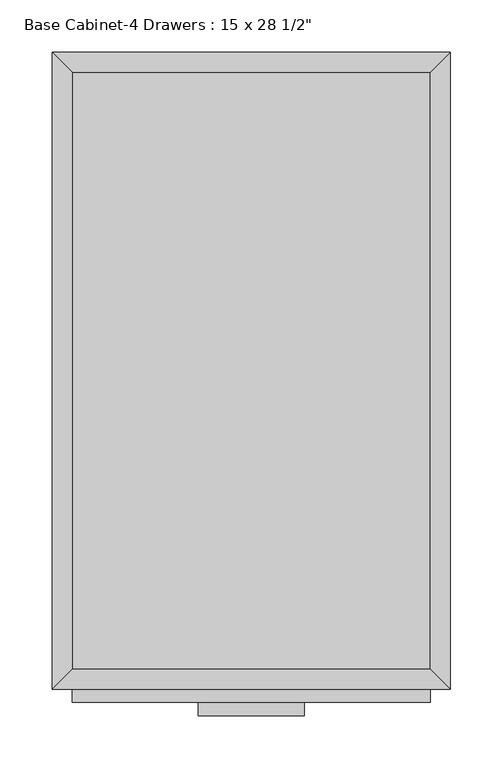
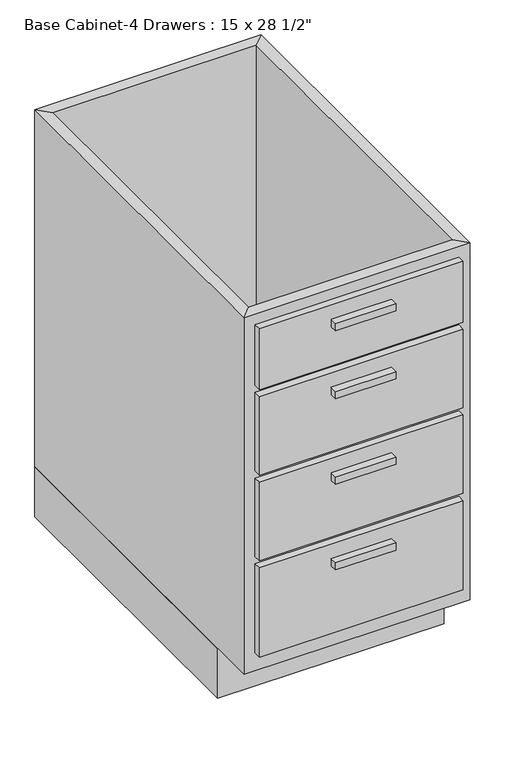
"""IFC4 building model written with IfcOpenShell, lengths in millimetres: furniture geometry."""

from ifc_helpers import new_model, si_unit, frame, origin, origin_with_axes, place, context, project, spatial, polyline, outline, extrude, faceted_brep, source, transform, mapped, element, save


def furniture_b6412ed0(model_context):
    return source(origin(), model_context, "Body", "SolidModel", [
        extrude(outline(polyline([(69.5377049, -635.0), (-32.0622951, -635.0), (-32.0622951, -622.3), (69.5377049, -622.3), (69.5377049, -635.0)])), frame((0.0, 0.0, 666.75), z_axis=(0.0, 0.0, 1.0), x_axis=(1.0, 0.0, 0.0)), (0.0, 0.0, 1.0), 12.7),
        extrude(outline(polyline([(69.5377049, -635.0), (-32.0622951, -635.0), (-32.0622951, -622.3), (69.5377049, -622.3), (69.5377049, -635.0)])), frame((0.0, 0.0, 546.1), z_axis=(0.0, 0.0, 1.0), x_axis=(1.0, 0.0, 0.0)), (0.0, 0.0, 1.0), 12.7),
        extrude(outline(polyline([(69.5377049, -635.0), (-32.0622951, -635.0), (-32.0622951, -622.3), (69.5377049, -622.3), (69.5377049, -635.0)])), frame((0.0, 0.0, 393.7), z_axis=(0.0, 0.0, 1.0), x_axis=(1.0, 0.0, 0.0)), (0.0, 0.0, 1.0), 12.7),
        extrude(outline(polyline([(69.5377049, -635.0), (-32.0622951, -635.0), (-32.0622951, -622.3), (69.5377049, -622.3), (69.5377049, -635.0)])), frame((0.0, 0.0, 241.3), z_axis=(0.0, 0.0, 1.0), x_axis=(1.0, 0.0, 0.0)), (0.0, 0.0, 1.0), 12.7),
        extrude(outline(polyline([(190.1877049, -622.3), (-152.7122951, -622.3), (-152.7122951, -609.6), (190.1877049, -609.6), (190.1877049, -622.3)])), frame((0.0, 0.0, 596.9), z_axis=(0.0, 0.0, 1.0), x_axis=(1.0, 0.0, 0.0)), (0.0, 0.0, 1.0), 107.95),
        extrude(outline(polyline([(190.1877049, -622.3), (-152.7122951, -622.3), (-152.7122951, -609.6), (190.1877049, -609.6), (190.1877049, -622.3)])), frame((0.0, 0.0, 444.5), z_axis=(0.0, 0.0, 1.0), x_axis=(1.0, 0.0, 0.0)), (0.0, 0.0, 1.0), 139.7),
        extrude(outline(polyline([(190.1877049, -622.3), (-152.7122951, -622.3), (-152.7122951, -609.6), (190.1877049, -609.6), (190.1877049, -622.3)])), frame((0.0, 0.0, 292.1), z_axis=(0.0, 0.0, 1.0), x_axis=(1.0, 0.0, 0.0)), (0.0, 0.0, 1.0), 139.7),
        extrude(outline(polyline([(190.1877049, -622.3), (-152.7122951, -622.3), (-152.7122951, -609.6), (190.1877049, -609.6), (190.1877049, -622.3)])), frame((0.0, 0.0, 120.65), z_axis=(0.0, 0.0, 1.0), x_axis=(1.0, 0.0, 0.0)), (0.0, 0.0, 1.0), 158.75),
        extrude(outline(polyline([(190.1877049, -19.05), (190.1877049, -590.55), (-152.7122951, -590.55), (-152.7122951, -19.05), (190.1877049, -19.05)])), frame((0.0, 0.0, 88.9), z_axis=(0.0, 0.0, 1.0), x_axis=(1.0, 0.0, 0.0)), (0.0, 0.0, 1.0), 19.05),
        faceted_brep([(190.1877049, -590.55, 723.9), (190.1877049, -590.55, 88.9), (-152.7122951, -590.55, 88.9), (-152.7122951, -590.55, 723.9), (209.2377049, -609.6, 723.9), (-171.7622951, -609.6, 723.9), (209.2377049, -609.6, 88.9), (-171.7622951, -609.6, 88.9), (-152.7122951, -19.05, 88.9), (-152.7122951, -19.05, 723.9), (-171.7622951, 0.0, 723.9), (-171.7622951, 0.0, 88.9), (190.1877049, -19.05, 88.9), (190.1877049, -19.05, 723.9), (209.2377049, 0.0, 723.9), (209.2377049, 0.0, 88.9)], [[[0, 1, 2, 3]], [[4, 0, 3, 5]], [[6, 4, 5, 7]], [[1, 6, 7, 2]], [[3, 2, 8, 9]], [[5, 3, 9, 10]], [[7, 5, 10, 11]], [[2, 7, 11, 8]], [[9, 8, 12, 13]], [[10, 9, 13, 14]], [[11, 10, 14, 15]], [[8, 11, 15, 12]], [[13, 12, 1, 0]], [[14, 13, 0, 4]], [[15, 14, 4, 6]], [[12, 15, 6, 1]]]),
        extrude(outline(polyline([(209.2377049, 0.0), (209.2377049, -533.4), (-171.7622951, -533.4), (-171.7622951, 0.0), (209.2377049, 0.0)])), origin_with_axes(), (0.0, 0.0, 1.0), 88.9),
    ])


if __name__ == "__main__":
    model = new_model("IFC4")
    model_context = context("Model", 3, world=origin())
    ifc_project = project(units=[si_unit("LENGTHUNIT", "METRE", prefix="MILLI")], contexts=[model_context])
    site = spatial("IfcSite", under=ifc_project)
    building = spatial("IfcBuilding", under=site)
    placement = place(None, origin())
    furniture_shape = furniture_b6412ed0(model_context)
    element("IfcFurniture", 1, ObjectType="Base Cabinet-4 Drawers : 15 x 28 1/2\"", at=placement, inside=building, context=model_context, shape_type="MappedRepresentation", body=[
        mapped(furniture_shape, transform((0.0, 0.0, 0.0), x_axis=(1.0, 0.0, 0.0), y_axis=(0.0, 1.0, 0.0), z_axis=(0.0, 0.0, 1.0))),
    ])
    save(model, "model.ifc")

# Revit data of these elements
# Type "Base Cabinet-4 Drawers : 15 x 28 1/2\""
#   COBie.Type.CreatedBy = "doug.wood@us.ibm.com"
#   COBie.Type.CreatedOn = "2016-04-14T02:07:23"
#   COBie.Type.Name = "Casework_Base Cabinet-4 Drawers_15 x 28 1/2\""
#   COBie.Type.Category = "23-40 35 17 47 11 : Kitchen Casework"
#   COBie.Type.Description = "Base Cabinet-4 Drawers_15 x 28 1/2\""
#   COBie.Type.Manufacturer = ""
#   COBie.Type.ModelNumber = ""
#   Assembly Code = "C1030410"
#   COBie.Type.ReplacementCost = 0
#   Depth = 2' - 0"
#   Height = 2' - 4 1/2"
#   Toe Depth = 0' - 3"
#   Toe Height = 0' - 3 1/2"
#   Width = 1' - 3"
#   COBie.Type = no
#   Cabinet Material = none
#   Door/Drawer Material = none
#   Handle Material = Cabinets - Handles
# Element 1 (IfcFurniture, "Base Cabinet-4 Drawers : 15 x 28 1/2\"")
#   Materials on its faces: "Cabinets", "Cabinets - Handles"
# Materials
#   "Cabinets - Handles": class "Metal", colour RGB 57 57 57, transparency 0
#   "Cabinets": class "Miscellaneous", colour RGB 249 249 249, transparency 0
